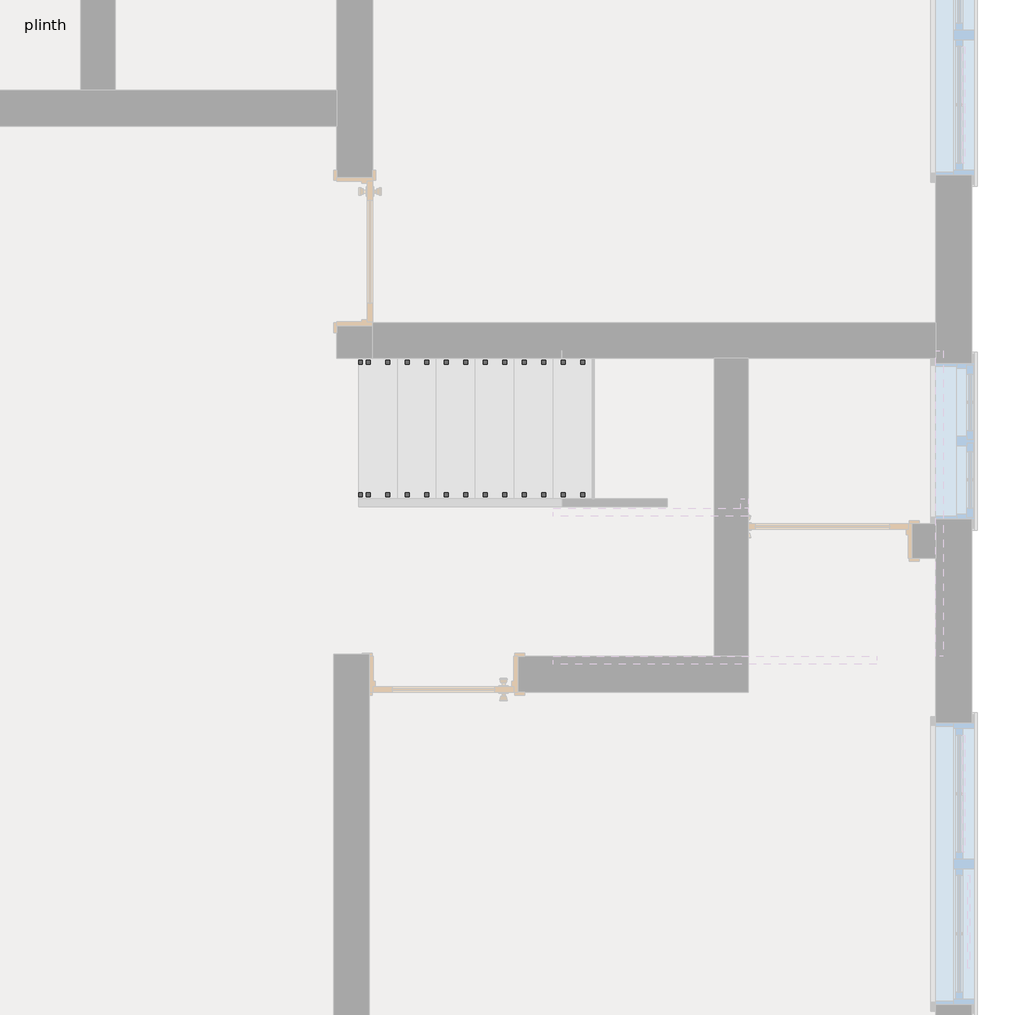
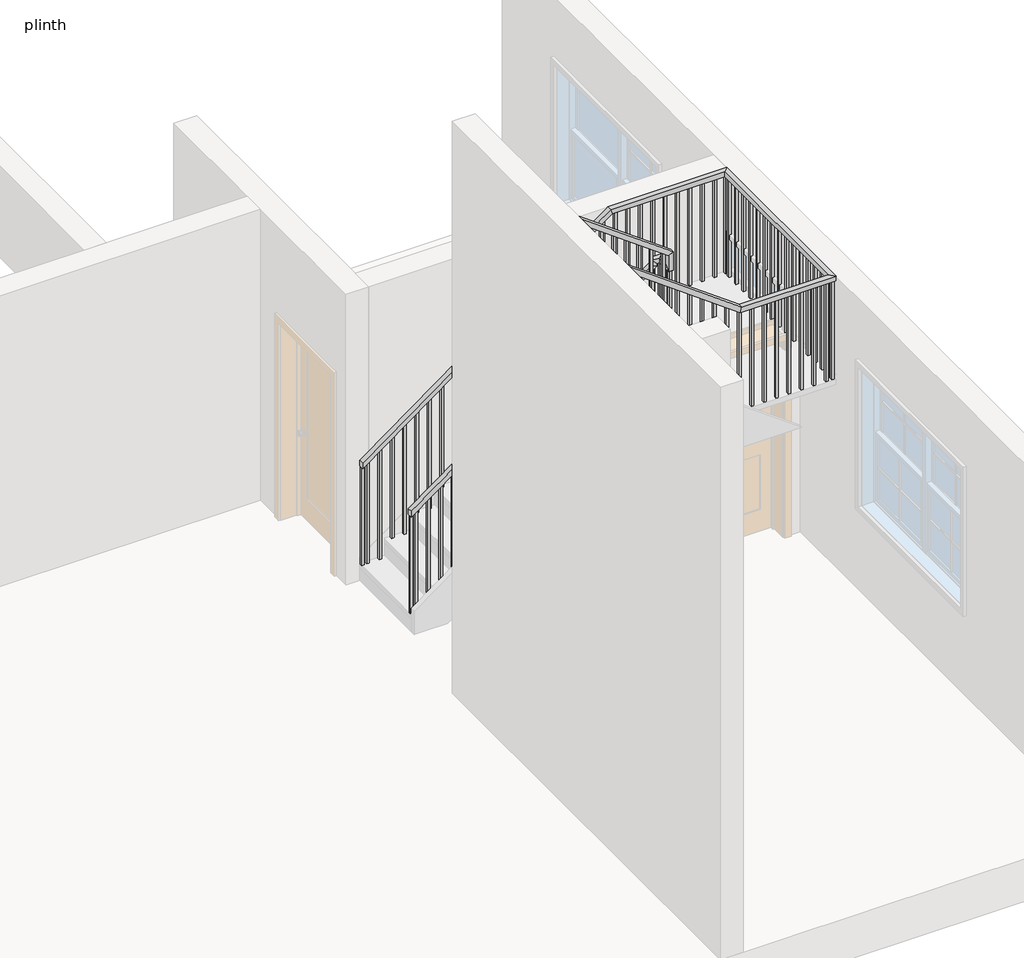
# One storey, part 2 of 3: 2 railings.
"""IFC4 building model written with IfcOpenShell, lengths in millimetres."""

from ifc_helpers import new_model, si_unit, frame, origin, place, context, project, spatial, polyline, outline, extrude, faceted_brep, element, save

model = new_model("IFC4")

# Units and contexts
model_context = context("Model", 3, world=origin())
ifc_project = project(units=[si_unit("LENGTHUNIT", "METRE", prefix="MILLI")], contexts=[model_context])

# Site, building, storey
site = spatial("IfcSite", under=ifc_project)
building = spatial("IfcBuilding", under=site)
storey = spatial("IfcBuildingStorey", under=building, Name="plinth", Elevation=450.0)

# Railings
placement = place(None, origin())
element("IfcRailing", 1, ObjectType="1100mm", at=placement, inside=storey, context=model_context, shape_type="SolidModel", body=[
    faceted_brep([(-8719.2253352, 6758.6914588, 1732.3529412), (-8719.2253352, 6758.6914588, 1670.4651087), (-8719.2253352, 6708.6914588, 1670.4651087), (-8719.2253352, 6708.6914588, 1732.3529412), (-6293.8253352, 6758.6914588, 3501.4682353), (-6243.8253352, 6758.6914588, 3476.0509911), (-6243.8253352, 6708.6914588, 3476.0509911), (-6293.8253352, 6708.6914588, 3501.4682353), (-6293.8253352, 6758.6914588, 3555.8823529), (-6243.8253352, 6758.6914588, 3505.8823529), (-6243.8253352, 6708.6914588, 3505.8823529), (-6293.8253352, 6708.6914588, 3555.8823529), (-6168.8253352, 6758.6914588, 3555.8823529), (-6168.8253352, 6758.6914588, 3505.8823529), (-6218.8253352, 6708.6914588, 3505.8823529), (-6218.8253352, 6708.6914588, 3555.8823529), (-6168.8253352, 6633.6914588, 3555.8823529), (-6168.8253352, 6633.6914588, 3505.8823529), (-6218.8253352, 6633.6914588, 3505.8823529), (-6218.8253352, 6633.6914588, 3555.8823529), (-6168.8253352, 6597.8914588, 3555.8823529), (-6218.8253352, 6597.8914588, 3555.8823529), (-6218.8253352, 6547.8914588, 3505.8823529), (-6168.8253352, 6547.8914588, 3505.8823529)], [[[0, 1, 2, 3]], [[1, 0, 4, 5]], [[2, 1, 5, 6]], [[3, 2, 6, 7]], [[0, 3, 7, 4]], [[5, 4, 8, 9]], [[6, 5, 9, 10]], [[7, 6, 10, 11]], [[4, 7, 11, 8]], [[9, 8, 12, 13]], [[10, 9, 13, 14]], [[11, 10, 14, 15]], [[8, 11, 15, 12]], [[13, 12, 16, 17]], [[14, 13, 17, 18]], [[15, 14, 18, 19]], [[12, 15, 19, 16]], [[20, 21, 22, 23]], [[17, 16, 20, 23]], [[18, 17, 23, 22]], [[19, 18, 22, 21]], [[16, 19, 21, 20]]]),
    faceted_brep([(-6168.8253352, 6597.8914588, 3555.8823529), (-6168.8253352, 6547.8914588, 3505.8823529), (-6218.8253352, 6547.8914588, 3505.8823529), (-6218.8253352, 6597.8914588, 3555.8823529), (-6168.8253352, 6597.8914588, 3701.4729412), (-6218.8253352, 6597.8914588, 3676.055697), (-6218.8253352, 6547.8914588, 3676.055697), (-6168.8253352, 6547.8914588, 3701.4729412)], [[[0, 1, 2, 3]], [[4, 5, 6, 7]], [[1, 0, 4, 7]], [[2, 1, 7, 6]], [[3, 2, 6, 5]], [[0, 3, 5, 4]]]),
    faceted_brep([(-6168.8253352, 6547.8914588, 3701.4729412), (-6218.8253352, 6547.8914588, 3676.055697), (-6218.8253352, 6597.8914588, 3676.055697), (-6168.8253352, 6597.8914588, 3701.4729412), (-7469.2253352, 6547.8914588, 4650.0), (-7469.2253352, 6597.8914588, 4650.0), (-7469.2253352, 6597.8914588, 4588.1121675), (-7469.2253352, 6547.8914588, 4588.1121675)], [[[0, 1, 2, 3]], [[4, 5, 6, 7]], [[1, 0, 4, 7]], [[2, 1, 7, 6]], [[3, 2, 6, 5]], [[0, 3, 5, 4]]]),
    extrude(outline(polyline([(3367.6470588, -7368.8253352), (4514.8792264, -7368.8253352), (4533.1145205, -7393.8253352), (3367.6470588, -7393.8253352), (3367.6470588, -7368.8253352)])), frame((0.0, 6560.3914588, 0.0), z_axis=(0.0, 1.0, 0.0), x_axis=(0.0, 0.0, 1.0)), (0.0, 0.0, 1.0), 25.0),
    extrude(outline(polyline([(3367.6470588, -7243.8253352), (4423.7027558, -7243.8253352), (4441.9380499, -7268.8253352), (3367.6470588, -7268.8253352), (3367.6470588, -7243.8253352)])), frame((0.0, 6560.3914588, 0.0), z_axis=(0.0, 1.0, 0.0), x_axis=(0.0, 0.0, 1.0)), (0.0, 0.0, 1.0), 25.0),
    extrude(outline(polyline([(3185.2941176, -7118.8253352), (4332.5262852, -7118.8253352), (4350.7615793, -7143.8253352), (3185.2941176, -7143.8253352), (3185.2941176, -7118.8253352)])), frame((0.0, 6560.3914588, 0.0), z_axis=(0.0, 1.0, 0.0), x_axis=(0.0, 0.0, 1.0)), (0.0, 0.0, 1.0), 25.0),
    extrude(outline(polyline([(3185.2941176, -6993.8253352), (4241.3498146, -6993.8253352), (4259.5851087, -7018.8253352), (3185.2941176, -7018.8253352), (3185.2941176, -6993.8253352)])), frame((0.0, 6560.3914588, 0.0), z_axis=(0.0, 1.0, 0.0), x_axis=(0.0, 0.0, 1.0)), (0.0, 0.0, 1.0), 25.0),
    extrude(outline(polyline([(3002.9411765, -6868.8253352), (4150.173344, -6868.8253352), (4168.4086381, -6893.8253352), (3002.9411765, -6893.8253352), (3002.9411765, -6868.8253352)])), frame((0.0, 6560.3914588, 0.0), z_axis=(0.0, 1.0, 0.0), x_axis=(0.0, 0.0, 1.0)), (0.0, 0.0, 1.0), 25.0),
    extrude(outline(polyline([(3002.9411765, -6743.8253352), (4058.9968734, -6743.8253352), (4077.2321675, -6768.8253352), (3002.9411765, -6768.8253352), (3002.9411765, -6743.8253352)])), frame((0.0, 6560.3914588, 0.0), z_axis=(0.0, 1.0, 0.0), x_axis=(0.0, 0.0, 1.0)), (0.0, 0.0, 1.0), 25.0),
    extrude(outline(polyline([(2820.5882353, -6618.8253352), (3967.8204028, -6618.8253352), (3986.055697, -6643.8253352), (2820.5882353, -6643.8253352), (2820.5882353, -6618.8253352)])), frame((0.0, 6560.3914588, 0.0), z_axis=(0.0, 1.0, 0.0), x_axis=(0.0, 0.0, 1.0)), (0.0, 0.0, 1.0), 25.0),
    extrude(outline(polyline([(2820.5882353, -6493.8253352), (3876.6439322, -6493.8253352), (3894.8792264, -6518.8253352), (2820.5882353, -6518.8253352), (2820.5882353, -6493.8253352)])), frame((0.0, 6560.3914588, 0.0), z_axis=(0.0, 1.0, 0.0), x_axis=(0.0, 0.0, 1.0)), (0.0, 0.0, 1.0), 25.0),
    extrude(outline(polyline([(2638.2352941, -6368.8253352), (3785.4674617, -6368.8253352), (3803.7027558, -6393.8253352), (2638.2352941, -6393.8253352), (2638.2352941, -6368.8253352)])), frame((0.0, 6560.3914588, 0.0), z_axis=(0.0, 1.0, 0.0), x_axis=(0.0, 0.0, 1.0)), (0.0, 0.0, 1.0), 25.0),
    extrude(outline(polyline([(2638.2352941, -6243.8253352), (3694.2909911, -6243.8253352), (3712.5262852, -6268.8253352), (2638.2352941, -6268.8253352), (2638.2352941, -6243.8253352)])), frame((0.0, 6560.3914588, 0.0), z_axis=(0.0, 1.0, 0.0), x_axis=(0.0, 0.0, 1.0)), (0.0, 0.0, 1.0), 25.0),
    extrude(outline(polyline([(-6206.3253352, 6683.6914588), (-6181.3253352, 6683.6914588), (-6181.3253352, 6658.6914588), (-6206.3253352, 6658.6914588), (-6206.3253352, 6683.6914588)])), frame((0.0, 0.0, 2455.8823529), z_axis=(0.0, 0.0, 1.0), x_axis=(1.0, 0.0, 0.0)), (0.0, 0.0, 1.0), 1050.0),
    extrude(outline(polyline([(-6294.2253352, 6721.1914588), (-6294.2253352, 6746.1914588), (-6269.2253352, 6746.1914588), (-6269.2253352, 6721.1914588), (-6294.2253352, 6721.1914588)])), frame((0.0, 0.0, 2273.5294118), z_axis=(0.0, 0.0, 1.0), x_axis=(1.0, 0.0, 0.0)), (0.0, 0.0, 1.0), 1232.3529412),
    extrude(outline(polyline([(3348.1121675, -6419.2253352), (2273.5294118, -6419.2253352), (2273.5294118, -6394.2253352), (3366.3474617, -6394.2253352), (3348.1121675, -6419.2253352)])), frame((0.0, 6721.1914588, 0.0), z_axis=(0.0, 1.0, 0.0), x_axis=(0.0, 0.0, 1.0)), (0.0, 0.0, 1.0), 25.0),
    extrude(outline(polyline([(3256.935697, -6544.2253352), (2091.1764706, -6544.2253352), (2091.1764706, -6519.2253352), (3275.1709911, -6519.2253352), (3256.935697, -6544.2253352)])), frame((0.0, 6721.1914588, 0.0), z_axis=(0.0, 1.0, 0.0), x_axis=(0.0, 0.0, 1.0)), (0.0, 0.0, 1.0), 25.0),
    extrude(outline(polyline([(3165.7592264, -6669.2253352), (2091.1764706, -6669.2253352), (2091.1764706, -6644.2253352), (3183.9945205, -6644.2253352), (3165.7592264, -6669.2253352)])), frame((0.0, 6721.1914588, 0.0), z_axis=(0.0, 1.0, 0.0), x_axis=(0.0, 0.0, 1.0)), (0.0, 0.0, 1.0), 25.0),
    extrude(outline(polyline([(3074.5827558, -6794.2253352), (1908.8235294, -6794.2253352), (1908.8235294, -6769.2253352), (3092.8180499, -6769.2253352), (3074.5827558, -6794.2253352)])), frame((0.0, 6721.1914588, 0.0), z_axis=(0.0, 1.0, 0.0), x_axis=(0.0, 0.0, 1.0)), (0.0, 0.0, 1.0), 25.0),
    extrude(outline(polyline([(2983.4062852, -6919.2253352), (1908.8235294, -6919.2253352), (1908.8235294, -6894.2253352), (3001.6415793, -6894.2253352), (2983.4062852, -6919.2253352)])), frame((0.0, 6721.1914588, 0.0), z_axis=(0.0, 1.0, 0.0), x_axis=(0.0, 0.0, 1.0)), (0.0, 0.0, 1.0), 25.0),
    extrude(outline(polyline([(2892.2298146, -7044.2253352), (1726.4705882, -7044.2253352), (1726.4705882, -7019.2253352), (2910.4651087, -7019.2253352), (2892.2298146, -7044.2253352)])), frame((0.0, 6721.1914588, 0.0), z_axis=(0.0, 1.0, 0.0), x_axis=(0.0, 0.0, 1.0)), (0.0, 0.0, 1.0), 25.0),
    extrude(outline(polyline([(2801.053344, -7169.2253352), (1726.4705882, -7169.2253352), (1726.4705882, -7144.2253352), (2819.2886381, -7144.2253352), (2801.053344, -7169.2253352)])), frame((0.0, 6721.1914588, 0.0), z_axis=(0.0, 1.0, 0.0), x_axis=(0.0, 0.0, 1.0)), (0.0, 0.0, 1.0), 25.0),
    extrude(outline(polyline([(2709.8768734, -7294.2253352), (1544.1176471, -7294.2253352), (1544.1176471, -7269.2253352), (2728.1121675, -7269.2253352), (2709.8768734, -7294.2253352)])), frame((0.0, 6721.1914588, 0.0), z_axis=(0.0, 1.0, 0.0), x_axis=(0.0, 0.0, 1.0)), (0.0, 0.0, 1.0), 25.0),
    extrude(outline(polyline([(2618.7004028, -7419.2253352), (1544.1176471, -7419.2253352), (1544.1176471, -7394.2253352), (2636.935697, -7394.2253352), (2618.7004028, -7419.2253352)])), frame((0.0, 6721.1914588, 0.0), z_axis=(0.0, 1.0, 0.0), x_axis=(0.0, 0.0, 1.0)), (0.0, 0.0, 1.0), 25.0),
    extrude(outline(polyline([(2527.5239322, -7544.2253352), (1361.7647059, -7544.2253352), (1361.7647059, -7519.2253352), (2545.7592264, -7519.2253352), (2527.5239322, -7544.2253352)])), frame((0.0, 6721.1914588, 0.0), z_axis=(0.0, 1.0, 0.0), x_axis=(0.0, 0.0, 1.0)), (0.0, 0.0, 1.0), 25.0),
    extrude(outline(polyline([(2436.3474617, -7669.2253352), (1361.7647059, -7669.2253352), (1361.7647059, -7644.2253352), (2454.5827558, -7644.2253352), (2436.3474617, -7669.2253352)])), frame((0.0, 6721.1914588, 0.0), z_axis=(0.0, 1.0, 0.0), x_axis=(0.0, 0.0, 1.0)), (0.0, 0.0, 1.0), 25.0),
    extrude(outline(polyline([(2345.1709911, -7794.2253352), (1179.4117647, -7794.2253352), (1179.4117647, -7769.2253352), (2363.4062852, -7769.2253352), (2345.1709911, -7794.2253352)])), frame((0.0, 6721.1914588, 0.0), z_axis=(0.0, 1.0, 0.0), x_axis=(0.0, 0.0, 1.0)), (0.0, 0.0, 1.0), 25.0),
    extrude(outline(polyline([(2253.9945205, -7919.2253352), (1179.4117647, -7919.2253352), (1179.4117647, -7894.2253352), (2272.2298146, -7894.2253352), (2253.9945205, -7919.2253352)])), frame((0.0, 6721.1914588, 0.0), z_axis=(0.0, 1.0, 0.0), x_axis=(0.0, 0.0, 1.0)), (0.0, 0.0, 1.0), 25.0),
    extrude(outline(polyline([(2162.8180499, -8044.2253352), (997.0588235, -8044.2253352), (997.0588235, -8019.2253352), (2181.053344, -8019.2253352), (2162.8180499, -8044.2253352)])), frame((0.0, 6721.1914588, 0.0), z_axis=(0.0, 1.0, 0.0), x_axis=(0.0, 0.0, 1.0)), (0.0, 0.0, 1.0), 25.0),
    extrude(outline(polyline([(2071.6415793, -8169.2253352), (997.0588235, -8169.2253352), (997.0588235, -8144.2253352), (2089.8768734, -8144.2253352), (2071.6415793, -8169.2253352)])), frame((0.0, 6721.1914588, 0.0), z_axis=(0.0, 1.0, 0.0), x_axis=(0.0, 0.0, 1.0)), (0.0, 0.0, 1.0), 25.0),
    extrude(outline(polyline([(1980.4651087, -8294.2253352), (814.7058824, -8294.2253352), (814.7058824, -8269.2253352), (1998.7004028, -8269.2253352), (1980.4651087, -8294.2253352)])), frame((0.0, 6721.1914588, 0.0), z_axis=(0.0, 1.0, 0.0), x_axis=(0.0, 0.0, 1.0)), (0.0, 0.0, 1.0), 25.0),
    extrude(outline(polyline([(1889.2886381, -8419.2253352), (814.7058824, -8419.2253352), (814.7058824, -8394.2253352), (1907.5239322, -8394.2253352), (1889.2886381, -8419.2253352)])), frame((0.0, 6721.1914588, 0.0), z_axis=(0.0, 1.0, 0.0), x_axis=(0.0, 0.0, 1.0)), (0.0, 0.0, 1.0), 25.0),
    extrude(outline(polyline([(1798.1121675, -8544.2253352), (632.3529412, -8544.2253352), (632.3529412, -8519.2253352), (1816.3474617, -8519.2253352), (1798.1121675, -8544.2253352)])), frame((0.0, 6721.1914588, 0.0), z_axis=(0.0, 1.0, 0.0), x_axis=(0.0, 0.0, 1.0)), (0.0, 0.0, 1.0), 25.0),
    extrude(outline(polyline([(1706.935697, -8669.2253352), (632.3529412, -8669.2253352), (632.3529412, -8644.2253352), (1725.1709911, -8644.2253352), (1706.935697, -8669.2253352)])), frame((0.0, 6721.1914588, 0.0), z_axis=(0.0, 1.0, 0.0), x_axis=(0.0, 0.0, 1.0)), (0.0, 0.0, 1.0), 25.0),
    extrude(outline(polyline([(-6206.3253352, 6585.3914588), (-6181.3253352, 6585.3914588), (-6181.3253352, 6560.3914588), (-6206.3253352, 6560.3914588), (-6206.3253352, 6585.3914588)])), frame((0.0, 0.0, 2455.8823529), z_axis=(0.0, 0.0, 1.0), x_axis=(1.0, 0.0, 0.0)), (0.0, 0.0, 1.0), 1050.0),
    extrude(outline(polyline([(-6206.3253352, 6721.1914588), (-6206.3253352, 6746.1914588), (-6181.3253352, 6746.1914588), (-6181.3253352, 6721.1914588), (-6206.3253352, 6721.1914588)])), frame((0.0, 0.0, 2455.8823529), z_axis=(0.0, 0.0, 1.0), x_axis=(1.0, 0.0, 0.0)), (0.0, 0.0, 1.0), 1050.0),
    extrude(outline(polyline([(3367.6470588, -7444.2253352), (4569.8768734, -7444.2253352), (4588.1121675, -7469.2253352), (3367.6470588, -7469.2253352), (3367.6470588, -7444.2253352)])), frame((0.0, 6560.3914588, 0.0), z_axis=(0.0, 1.0, 0.0), x_axis=(0.0, 0.0, 1.0)), (0.0, 0.0, 1.0), 25.0),
    extrude(outline(polyline([(1670.4651087, -8719.2253352), (632.3529412, -8719.2253352), (632.3529412, -8694.2253352), (1688.7004028, -8694.2253352), (1670.4651087, -8719.2253352)])), frame((0.0, 6721.1914588, 0.0), z_axis=(0.0, 1.0, 0.0), x_axis=(0.0, 0.0, 1.0)), (0.0, 0.0, 1.0), 25.0),
])
element("IfcRailing", 2, ObjectType="1100mm", at=placement, inside=storey, context=model_context, shape_type="SolidModel", body=[
    faceted_brep([(-8719.2253352, 7607.8914588, 1732.3529412), (-8719.2253352, 7607.8914588, 1670.4651087), (-8719.2253352, 7557.8914588, 1670.4651087), (-8719.2253352, 7557.8914588, 1732.3529412), (-6219.2253352, 7607.8914588, 3555.8823529), (-6202.9275004, 7607.8914588, 3505.8823529), (-6202.9275004, 7557.8914588, 3505.8823529), (-6219.2253352, 7557.8914588, 3555.8823529), (-5019.6253352, 7607.8914588, 3555.8823529), (-5019.6253352, 7607.8914588, 3505.8823529), (-5069.6253352, 7557.8914588, 3505.8823529), (-5069.6253352, 7557.8914588, 3555.8823529), (-5019.6253352, 5698.6914588, 3555.8823529), (-5019.6253352, 5698.6914588, 3505.8823529), (-5069.6253352, 5748.6914588, 3505.8823529), (-5069.6253352, 5748.6914588, 3555.8823529), (-5969.2253352, 5698.6914588, 3555.8823529), (-5985.52317, 5698.6914588, 3505.8823529), (-5985.52317, 5748.6914588, 3505.8823529), (-5969.2253352, 5748.6914588, 3555.8823529), (-7469.2253352, 5698.6914588, 4650.0), (-7469.2253352, 5748.6914588, 4650.0), (-7469.2253352, 5748.6914588, 4588.1121675), (-7469.2253352, 5698.6914588, 4588.1121675)], [[[0, 1, 2, 3]], [[1, 0, 4, 5]], [[2, 1, 5, 6]], [[3, 2, 6, 7]], [[0, 3, 7, 4]], [[5, 4, 8, 9]], [[6, 5, 9, 10]], [[7, 6, 10, 11]], [[4, 7, 11, 8]], [[9, 8, 12, 13]], [[10, 9, 13, 14]], [[11, 10, 14, 15]], [[8, 11, 15, 12]], [[13, 12, 16, 17]], [[14, 13, 17, 18]], [[15, 14, 18, 19]], [[12, 15, 19, 16]], [[20, 21, 22, 23]], [[17, 16, 20, 23]], [[18, 17, 23, 22]], [[19, 18, 22, 21]], [[16, 19, 21, 20]]]),
    extrude(outline(polyline([(4497.2274617, -7344.6253352), (4515.4627558, -7369.6253352), (3367.6470588, -7369.6253352), (3367.6470588, -7344.6253352), (4497.2274617, -7344.6253352)])), frame((0.0, 5711.1914588, 0.0), z_axis=(0.0, 1.0, 0.0), x_axis=(0.0, 0.0, 1.0)), (0.0, 0.0, 1.0), 25.0),
    extrude(outline(polyline([(4406.0509911, -7219.6253352), (4424.2862852, -7244.6253352), (3367.6470588, -7244.6253352), (3367.6470588, -7219.6253352), (4406.0509911, -7219.6253352)])), frame((0.0, 5711.1914588, 0.0), z_axis=(0.0, 1.0, 0.0), x_axis=(0.0, 0.0, 1.0)), (0.0, 0.0, 1.0), 25.0),
    extrude(outline(polyline([(4314.8745205, -7094.6253352), (4333.1098146, -7119.6253352), (3185.2941176, -7119.6253352), (3185.2941176, -7094.6253352), (4314.8745205, -7094.6253352)])), frame((0.0, 5711.1914588, 0.0), z_axis=(0.0, 1.0, 0.0), x_axis=(0.0, 0.0, 1.0)), (0.0, 0.0, 1.0), 25.0),
    extrude(outline(polyline([(4223.6980499, -6969.6253352), (4241.933344, -6994.6253352), (3185.2941176, -6994.6253352), (3185.2941176, -6969.6253352), (4223.6980499, -6969.6253352)])), frame((0.0, 5711.1914588, 0.0), z_axis=(0.0, 1.0, 0.0), x_axis=(0.0, 0.0, 1.0)), (0.0, 0.0, 1.0), 25.0),
    extrude(outline(polyline([(4132.5215793, -6844.6253352), (4150.7568734, -6869.6253352), (3002.9411765, -6869.6253352), (3002.9411765, -6844.6253352), (4132.5215793, -6844.6253352)])), frame((0.0, 5711.1914588, 0.0), z_axis=(0.0, 1.0, 0.0), x_axis=(0.0, 0.0, 1.0)), (0.0, 0.0, 1.0), 25.0),
    extrude(outline(polyline([(4041.3451087, -6719.6253352), (4059.5804028, -6744.6253352), (3002.9411765, -6744.6253352), (3002.9411765, -6719.6253352), (4041.3451087, -6719.6253352)])), frame((0.0, 5711.1914588, 0.0), z_axis=(0.0, 1.0, 0.0), x_axis=(0.0, 0.0, 1.0)), (0.0, 0.0, 1.0), 25.0),
    extrude(outline(polyline([(3950.1686381, -6594.6253352), (3968.4039322, -6619.6253352), (2820.5882353, -6619.6253352), (2820.5882353, -6594.6253352), (3950.1686381, -6594.6253352)])), frame((0.0, 5711.1914588, 0.0), z_axis=(0.0, 1.0, 0.0), x_axis=(0.0, 0.0, 1.0)), (0.0, 0.0, 1.0), 25.0),
    extrude(outline(polyline([(3858.9921675, -6469.6253352), (3877.2274617, -6494.6253352), (2820.5882353, -6494.6253352), (2820.5882353, -6469.6253352), (3858.9921675, -6469.6253352)])), frame((0.0, 5711.1914588, 0.0), z_axis=(0.0, 1.0, 0.0), x_axis=(0.0, 0.0, 1.0)), (0.0, 0.0, 1.0), 25.0),
    extrude(outline(polyline([(3767.815697, -6344.6253352), (3786.0509911, -6369.6253352), (2638.2352941, -6369.6253352), (2638.2352941, -6344.6253352), (3767.815697, -6344.6253352)])), frame((0.0, 5711.1914588, 0.0), z_axis=(0.0, 1.0, 0.0), x_axis=(0.0, 0.0, 1.0)), (0.0, 0.0, 1.0), 25.0),
    extrude(outline(polyline([(3676.6392264, -6219.6253352), (3694.8745205, -6244.6253352), (2638.2352941, -6244.6253352), (2638.2352941, -6219.6253352), (3676.6392264, -6219.6253352)])), frame((0.0, 5711.1914588, 0.0), z_axis=(0.0, 1.0, 0.0), x_axis=(0.0, 0.0, 1.0)), (0.0, 0.0, 1.0), 25.0),
    extrude(outline(polyline([(3585.4627558, -6094.6253352), (3603.6980499, -6119.6253352), (2455.8823529, -6119.6253352), (2455.8823529, -6094.6253352), (3585.4627558, -6094.6253352)])), frame((0.0, 5711.1914588, 0.0), z_axis=(0.0, 1.0, 0.0), x_axis=(0.0, 0.0, 1.0)), (0.0, 0.0, 1.0), 25.0),
    extrude(outline(polyline([(3494.2862852, -5969.6253352), (3512.5215793, -5994.6253352), (2455.8823529, -5994.6253352), (2455.8823529, -5969.6253352), (3494.2862852, -5969.6253352)])), frame((0.0, 5711.1914588, 0.0), z_axis=(0.0, 1.0, 0.0), x_axis=(0.0, 0.0, 1.0)), (0.0, 0.0, 1.0), 25.0),
    extrude(outline(polyline([(-5844.6253352, 5711.1914588), (-5869.6253352, 5711.1914588), (-5869.6253352, 5736.1914588), (-5844.6253352, 5736.1914588), (-5844.6253352, 5711.1914588)])), frame((0.0, 0.0, 2455.8823529), z_axis=(0.0, 0.0, 1.0), x_axis=(1.0, 0.0, 0.0)), (0.0, 0.0, 1.0), 1050.0),
    extrude(outline(polyline([(-5719.6253352, 5711.1914588), (-5744.6253352, 5711.1914588), (-5744.6253352, 5736.1914588), (-5719.6253352, 5736.1914588), (-5719.6253352, 5711.1914588)])), frame((0.0, 0.0, 2455.8823529), z_axis=(0.0, 0.0, 1.0), x_axis=(1.0, 0.0, 0.0)), (0.0, 0.0, 1.0), 1050.0),
    extrude(outline(polyline([(-5594.6253352, 5711.1914588), (-5619.6253352, 5711.1914588), (-5619.6253352, 5736.1914588), (-5594.6253352, 5736.1914588), (-5594.6253352, 5711.1914588)])), frame((0.0, 0.0, 2455.8823529), z_axis=(0.0, 0.0, 1.0), x_axis=(1.0, 0.0, 0.0)), (0.0, 0.0, 1.0), 1050.0),
    extrude(outline(polyline([(-5469.6253352, 5711.1914588), (-5494.6253352, 5711.1914588), (-5494.6253352, 5736.1914588), (-5469.6253352, 5736.1914588), (-5469.6253352, 5711.1914588)])), frame((0.0, 0.0, 2455.8823529), z_axis=(0.0, 0.0, 1.0), x_axis=(1.0, 0.0, 0.0)), (0.0, 0.0, 1.0), 1050.0),
    extrude(outline(polyline([(-5344.6253352, 5711.1914588), (-5369.6253352, 5711.1914588), (-5369.6253352, 5736.1914588), (-5344.6253352, 5736.1914588), (-5344.6253352, 5711.1914588)])), frame((0.0, 0.0, 2455.8823529), z_axis=(0.0, 0.0, 1.0), x_axis=(1.0, 0.0, 0.0)), (0.0, 0.0, 1.0), 1050.0),
    extrude(outline(polyline([(-5219.6253352, 5711.1914588), (-5244.6253352, 5711.1914588), (-5244.6253352, 5736.1914588), (-5219.6253352, 5736.1914588), (-5219.6253352, 5711.1914588)])), frame((0.0, 0.0, 2455.8823529), z_axis=(0.0, 0.0, 1.0), x_axis=(1.0, 0.0, 0.0)), (0.0, 0.0, 1.0), 1050.0),
    extrude(outline(polyline([(-5094.6253352, 5711.1914588), (-5119.6253352, 5711.1914588), (-5119.6253352, 5736.1914588), (-5094.6253352, 5736.1914588), (-5094.6253352, 5711.1914588)])), frame((0.0, 0.0, 2455.8823529), z_axis=(0.0, 0.0, 1.0), x_axis=(1.0, 0.0, 0.0)), (0.0, 0.0, 1.0), 1050.0),
    extrude(outline(polyline([(-5032.1253352, 5782.8914588), (-5032.1253352, 5757.8914588), (-5057.1253352, 5757.8914588), (-5057.1253352, 5782.8914588), (-5032.1253352, 5782.8914588)])), frame((0.0, 0.0, 2455.8823529), z_axis=(0.0, 0.0, 1.0), x_axis=(1.0, 0.0, 0.0)), (0.0, 0.0, 1.0), 1050.0),
    extrude(outline(polyline([(-5032.1253352, 5907.8914588), (-5032.1253352, 5882.8914588), (-5057.1253352, 5882.8914588), (-5057.1253352, 5907.8914588), (-5032.1253352, 5907.8914588)])), frame((0.0, 0.0, 2455.8823529), z_axis=(0.0, 0.0, 1.0), x_axis=(1.0, 0.0, 0.0)), (0.0, 0.0, 1.0), 1050.0),
    extrude(outline(polyline([(-5032.1253352, 6032.8914588), (-5032.1253352, 6007.8914588), (-5057.1253352, 6007.8914588), (-5057.1253352, 6032.8914588), (-5032.1253352, 6032.8914588)])), frame((0.0, 0.0, 2455.8823529), z_axis=(0.0, 0.0, 1.0), x_axis=(1.0, 0.0, 0.0)), (0.0, 0.0, 1.0), 1050.0),
    extrude(outline(polyline([(-5032.1253352, 6157.8914588), (-5032.1253352, 6132.8914588), (-5057.1253352, 6132.8914588), (-5057.1253352, 6157.8914588), (-5032.1253352, 6157.8914588)])), frame((0.0, 0.0, 2455.8823529), z_axis=(0.0, 0.0, 1.0), x_axis=(1.0, 0.0, 0.0)), (0.0, 0.0, 1.0), 1050.0),
    extrude(outline(polyline([(-5032.1253352, 6282.8914588), (-5032.1253352, 6257.8914588), (-5057.1253352, 6257.8914588), (-5057.1253352, 6282.8914588), (-5032.1253352, 6282.8914588)])), frame((0.0, 0.0, 2455.8823529), z_axis=(0.0, 0.0, 1.0), x_axis=(1.0, 0.0, 0.0)), (0.0, 0.0, 1.0), 1050.0),
    extrude(outline(polyline([(-5032.1253352, 6407.8914588), (-5032.1253352, 6382.8914588), (-5057.1253352, 6382.8914588), (-5057.1253352, 6407.8914588), (-5032.1253352, 6407.8914588)])), frame((0.0, 0.0, 2455.8823529), z_axis=(0.0, 0.0, 1.0), x_axis=(1.0, 0.0, 0.0)), (0.0, 0.0, 1.0), 1050.0),
    extrude(outline(polyline([(-5032.1253352, 6532.8914588), (-5032.1253352, 6507.8914588), (-5057.1253352, 6507.8914588), (-5057.1253352, 6532.8914588), (-5032.1253352, 6532.8914588)])), frame((0.0, 0.0, 2455.8823529), z_axis=(0.0, 0.0, 1.0), x_axis=(1.0, 0.0, 0.0)), (0.0, 0.0, 1.0), 1050.0),
    extrude(outline(polyline([(-5032.1253352, 6657.8914588), (-5032.1253352, 6632.8914588), (-5057.1253352, 6632.8914588), (-5057.1253352, 6657.8914588), (-5032.1253352, 6657.8914588)])), frame((0.0, 0.0, 2455.8823529), z_axis=(0.0, 0.0, 1.0), x_axis=(1.0, 0.0, 0.0)), (0.0, 0.0, 1.0), 1050.0),
    extrude(outline(polyline([(-5032.1253352, 6782.8914588), (-5032.1253352, 6757.8914588), (-5057.1253352, 6757.8914588), (-5057.1253352, 6782.8914588), (-5032.1253352, 6782.8914588)])), frame((0.0, 0.0, 2455.8823529), z_axis=(0.0, 0.0, 1.0), x_axis=(1.0, 0.0, 0.0)), (0.0, 0.0, 1.0), 1050.0),
    extrude(outline(polyline([(-5032.1253352, 6907.8914588), (-5032.1253352, 6882.8914588), (-5057.1253352, 6882.8914588), (-5057.1253352, 6907.8914588), (-5032.1253352, 6907.8914588)])), frame((0.0, 0.0, 2455.8823529), z_axis=(0.0, 0.0, 1.0), x_axis=(1.0, 0.0, 0.0)), (0.0, 0.0, 1.0), 1050.0),
    extrude(outline(polyline([(-5032.1253352, 7032.8914588), (-5032.1253352, 7007.8914588), (-5057.1253352, 7007.8914588), (-5057.1253352, 7032.8914588), (-5032.1253352, 7032.8914588)])), frame((0.0, 0.0, 2455.8823529), z_axis=(0.0, 0.0, 1.0), x_axis=(1.0, 0.0, 0.0)), (0.0, 0.0, 1.0), 1050.0),
    extrude(outline(polyline([(-5032.1253352, 7157.8914588), (-5032.1253352, 7132.8914588), (-5057.1253352, 7132.8914588), (-5057.1253352, 7157.8914588), (-5032.1253352, 7157.8914588)])), frame((0.0, 0.0, 2455.8823529), z_axis=(0.0, 0.0, 1.0), x_axis=(1.0, 0.0, 0.0)), (0.0, 0.0, 1.0), 1050.0),
    extrude(outline(polyline([(-5032.1253352, 7282.8914588), (-5032.1253352, 7257.8914588), (-5057.1253352, 7257.8914588), (-5057.1253352, 7282.8914588), (-5032.1253352, 7282.8914588)])), frame((0.0, 0.0, 2455.8823529), z_axis=(0.0, 0.0, 1.0), x_axis=(1.0, 0.0, 0.0)), (0.0, 0.0, 1.0), 1050.0),
    extrude(outline(polyline([(-5032.1253352, 7407.8914588), (-5032.1253352, 7382.8914588), (-5057.1253352, 7382.8914588), (-5057.1253352, 7407.8914588), (-5032.1253352, 7407.8914588)])), frame((0.0, 0.0, 2455.8823529), z_axis=(0.0, 0.0, 1.0), x_axis=(1.0, 0.0, 0.0)), (0.0, 0.0, 1.0), 1050.0),
    extrude(outline(polyline([(-5032.1253352, 7532.8914588), (-5032.1253352, 7507.8914588), (-5057.1253352, 7507.8914588), (-5057.1253352, 7532.8914588), (-5032.1253352, 7532.8914588)])), frame((0.0, 0.0, 2455.8823529), z_axis=(0.0, 0.0, 1.0), x_axis=(1.0, 0.0, 0.0)), (0.0, 0.0, 1.0), 1050.0),
    extrude(outline(polyline([(-5169.2253352, 7595.3914588), (-5144.2253352, 7595.3914588), (-5144.2253352, 7570.3914588), (-5169.2253352, 7570.3914588), (-5169.2253352, 7595.3914588)])), frame((0.0, 0.0, 2455.8823529), z_axis=(0.0, 0.0, 1.0), x_axis=(1.0, 0.0, 0.0)), (0.0, 0.0, 1.0), 1050.0),
    extrude(outline(polyline([(-5294.2253352, 7595.3914588), (-5269.2253352, 7595.3914588), (-5269.2253352, 7570.3914588), (-5294.2253352, 7570.3914588), (-5294.2253352, 7595.3914588)])), frame((0.0, 0.0, 2455.8823529), z_axis=(0.0, 0.0, 1.0), x_axis=(1.0, 0.0, 0.0)), (0.0, 0.0, 1.0), 1050.0),
    extrude(outline(polyline([(-5419.2253352, 7595.3914588), (-5394.2253352, 7595.3914588), (-5394.2253352, 7570.3914588), (-5419.2253352, 7570.3914588), (-5419.2253352, 7595.3914588)])), frame((0.0, 0.0, 2455.8823529), z_axis=(0.0, 0.0, 1.0), x_axis=(1.0, 0.0, 0.0)), (0.0, 0.0, 1.0), 1050.0),
    extrude(outline(polyline([(-5544.2253352, 7595.3914588), (-5519.2253352, 7595.3914588), (-5519.2253352, 7570.3914588), (-5544.2253352, 7570.3914588), (-5544.2253352, 7595.3914588)])), frame((0.0, 0.0, 2455.8823529), z_axis=(0.0, 0.0, 1.0), x_axis=(1.0, 0.0, 0.0)), (0.0, 0.0, 1.0), 1050.0),
    extrude(outline(polyline([(-5669.2253352, 7595.3914588), (-5644.2253352, 7595.3914588), (-5644.2253352, 7570.3914588), (-5669.2253352, 7570.3914588), (-5669.2253352, 7595.3914588)])), frame((0.0, 0.0, 2455.8823529), z_axis=(0.0, 0.0, 1.0), x_axis=(1.0, 0.0, 0.0)), (0.0, 0.0, 1.0), 1050.0),
    extrude(outline(polyline([(-5794.2253352, 7595.3914588), (-5769.2253352, 7595.3914588), (-5769.2253352, 7570.3914588), (-5794.2253352, 7570.3914588), (-5794.2253352, 7595.3914588)])), frame((0.0, 0.0, 2455.8823529), z_axis=(0.0, 0.0, 1.0), x_axis=(1.0, 0.0, 0.0)), (0.0, 0.0, 1.0), 1050.0),
    extrude(outline(polyline([(-5919.2253352, 7595.3914588), (-5894.2253352, 7595.3914588), (-5894.2253352, 7570.3914588), (-5919.2253352, 7570.3914588), (-5919.2253352, 7595.3914588)])), frame((0.0, 0.0, 2455.8823529), z_axis=(0.0, 0.0, 1.0), x_axis=(1.0, 0.0, 0.0)), (0.0, 0.0, 1.0), 1050.0),
    extrude(outline(polyline([(-6044.2253352, 7595.3914588), (-6019.2253352, 7595.3914588), (-6019.2253352, 7570.3914588), (-6044.2253352, 7570.3914588), (-6044.2253352, 7595.3914588)])), frame((0.0, 0.0, 2455.8823529), z_axis=(0.0, 0.0, 1.0), x_axis=(1.0, 0.0, 0.0)), (0.0, 0.0, 1.0), 1050.0),
    extrude(outline(polyline([(-6169.2253352, 7595.3914588), (-6144.2253352, 7595.3914588), (-6144.2253352, 7570.3914588), (-6169.2253352, 7570.3914588), (-6169.2253352, 7595.3914588)])), frame((0.0, 0.0, 2455.8823529), z_axis=(0.0, 0.0, 1.0), x_axis=(1.0, 0.0, 0.0)), (0.0, 0.0, 1.0), 1050.0),
    extrude(outline(polyline([(2273.5294118, -6294.2253352), (2273.5294118, -6269.2253352), (3457.5239322, -6269.2253352), (3439.2886381, -6294.2253352), (2273.5294118, -6294.2253352)])), frame((0.0, 7570.3914588, 0.0), z_axis=(0.0, 1.0, 0.0), x_axis=(0.0, 0.0, 1.0)), (0.0, 0.0, 1.0), 25.0),
    extrude(outline(polyline([(2273.5294118, -6419.2253352), (2273.5294118, -6394.2253352), (3366.3474617, -6394.2253352), (3348.1121675, -6419.2253352), (2273.5294118, -6419.2253352)])), frame((0.0, 7570.3914588, 0.0), z_axis=(0.0, 1.0, 0.0), x_axis=(0.0, 0.0, 1.0)), (0.0, 0.0, 1.0), 25.0),
    extrude(outline(polyline([(2091.1764706, -6544.2253352), (2091.1764706, -6519.2253352), (3275.1709911, -6519.2253352), (3256.935697, -6544.2253352), (2091.1764706, -6544.2253352)])), frame((0.0, 7570.3914588, 0.0), z_axis=(0.0, 1.0, 0.0), x_axis=(0.0, 0.0, 1.0)), (0.0, 0.0, 1.0), 25.0),
    extrude(outline(polyline([(2091.1764706, -6669.2253352), (2091.1764706, -6644.2253352), (3183.9945205, -6644.2253352), (3165.7592264, -6669.2253352), (2091.1764706, -6669.2253352)])), frame((0.0, 7570.3914588, 0.0), z_axis=(0.0, 1.0, 0.0), x_axis=(0.0, 0.0, 1.0)), (0.0, 0.0, 1.0), 25.0),
    extrude(outline(polyline([(1908.8235294, -6794.2253352), (1908.8235294, -6769.2253352), (3092.8180499, -6769.2253352), (3074.5827558, -6794.2253352), (1908.8235294, -6794.2253352)])), frame((0.0, 7570.3914588, 0.0), z_axis=(0.0, 1.0, 0.0), x_axis=(0.0, 0.0, 1.0)), (0.0, 0.0, 1.0), 25.0),
    extrude(outline(polyline([(1908.8235294, -6919.2253352), (1908.8235294, -6894.2253352), (3001.6415793, -6894.2253352), (2983.4062852, -6919.2253352), (1908.8235294, -6919.2253352)])), frame((0.0, 7570.3914588, 0.0), z_axis=(0.0, 1.0, 0.0), x_axis=(0.0, 0.0, 1.0)), (0.0, 0.0, 1.0), 25.0),
    extrude(outline(polyline([(1726.4705882, -7044.2253352), (1726.4705882, -7019.2253352), (2910.4651087, -7019.2253352), (2892.2298146, -7044.2253352), (1726.4705882, -7044.2253352)])), frame((0.0, 7570.3914588, 0.0), z_axis=(0.0, 1.0, 0.0), x_axis=(0.0, 0.0, 1.0)), (0.0, 0.0, 1.0), 25.0),
    extrude(outline(polyline([(1726.4705882, -7169.2253352), (1726.4705882, -7144.2253352), (2819.2886381, -7144.2253352), (2801.053344, -7169.2253352), (1726.4705882, -7169.2253352)])), frame((0.0, 7570.3914588, 0.0), z_axis=(0.0, 1.0, 0.0), x_axis=(0.0, 0.0, 1.0)), (0.0, 0.0, 1.0), 25.0),
    extrude(outline(polyline([(1544.1176471, -7294.2253352), (1544.1176471, -7269.2253352), (2728.1121675, -7269.2253352), (2709.8768734, -7294.2253352), (1544.1176471, -7294.2253352)])), frame((0.0, 7570.3914588, 0.0), z_axis=(0.0, 1.0, 0.0), x_axis=(0.0, 0.0, 1.0)), (0.0, 0.0, 1.0), 25.0),
    extrude(outline(polyline([(1544.1176471, -7419.2253352), (1544.1176471, -7394.2253352), (2636.935697, -7394.2253352), (2618.7004028, -7419.2253352), (1544.1176471, -7419.2253352)])), frame((0.0, 7570.3914588, 0.0), z_axis=(0.0, 1.0, 0.0), x_axis=(0.0, 0.0, 1.0)), (0.0, 0.0, 1.0), 25.0),
    extrude(outline(polyline([(1361.7647059, -7544.2253352), (1361.7647059, -7519.2253352), (2545.7592264, -7519.2253352), (2527.5239322, -7544.2253352), (1361.7647059, -7544.2253352)])), frame((0.0, 7570.3914588, 0.0), z_axis=(0.0, 1.0, 0.0), x_axis=(0.0, 0.0, 1.0)), (0.0, 0.0, 1.0), 25.0),
    extrude(outline(polyline([(1361.7647059, -7669.2253352), (1361.7647059, -7644.2253352), (2454.5827558, -7644.2253352), (2436.3474617, -7669.2253352), (1361.7647059, -7669.2253352)])), frame((0.0, 7570.3914588, 0.0), z_axis=(0.0, 1.0, 0.0), x_axis=(0.0, 0.0, 1.0)), (0.0, 0.0, 1.0), 25.0),
    extrude(outline(polyline([(1179.4117647, -7794.2253352), (1179.4117647, -7769.2253352), (2363.4062852, -7769.2253352), (2345.1709911, -7794.2253352), (1179.4117647, -7794.2253352)])), frame((0.0, 7570.3914588, 0.0), z_axis=(0.0, 1.0, 0.0), x_axis=(0.0, 0.0, 1.0)), (0.0, 0.0, 1.0), 25.0),
    extrude(outline(polyline([(1179.4117647, -7919.2253352), (1179.4117647, -7894.2253352), (2272.2298146, -7894.2253352), (2253.9945205, -7919.2253352), (1179.4117647, -7919.2253352)])), frame((0.0, 7570.3914588, 0.0), z_axis=(0.0, 1.0, 0.0), x_axis=(0.0, 0.0, 1.0)), (0.0, 0.0, 1.0), 25.0),
    extrude(outline(polyline([(997.0588235, -8044.2253352), (997.0588235, -8019.2253352), (2181.053344, -8019.2253352), (2162.8180499, -8044.2253352), (997.0588235, -8044.2253352)])), frame((0.0, 7570.3914588, 0.0), z_axis=(0.0, 1.0, 0.0), x_axis=(0.0, 0.0, 1.0)), (0.0, 0.0, 1.0), 25.0),
    extrude(outline(polyline([(997.0588235, -8169.2253352), (997.0588235, -8144.2253352), (2089.8768734, -8144.2253352), (2071.6415793, -8169.2253352), (997.0588235, -8169.2253352)])), frame((0.0, 7570.3914588, 0.0), z_axis=(0.0, 1.0, 0.0), x_axis=(0.0, 0.0, 1.0)), (0.0, 0.0, 1.0), 25.0),
    extrude(outline(polyline([(814.7058824, -8294.2253352), (814.7058824, -8269.2253352), (1998.7004028, -8269.2253352), (1980.4651087, -8294.2253352), (814.7058824, -8294.2253352)])), frame((0.0, 7570.3914588, 0.0), z_axis=(0.0, 1.0, 0.0), x_axis=(0.0, 0.0, 1.0)), (0.0, 0.0, 1.0), 25.0),
    extrude(outline(polyline([(814.7058824, -8419.2253352), (814.7058824, -8394.2253352), (1907.5239322, -8394.2253352), (1889.2886381, -8419.2253352), (814.7058824, -8419.2253352)])), frame((0.0, 7570.3914588, 0.0), z_axis=(0.0, 1.0, 0.0), x_axis=(0.0, 0.0, 1.0)), (0.0, 0.0, 1.0), 25.0),
    extrude(outline(polyline([(632.3529412, -8544.2253352), (632.3529412, -8519.2253352), (1816.3474617, -8519.2253352), (1798.1121675, -8544.2253352), (632.3529412, -8544.2253352)])), frame((0.0, 7570.3914588, 0.0), z_axis=(0.0, 1.0, 0.0), x_axis=(0.0, 0.0, 1.0)), (0.0, 0.0, 1.0), 25.0),
    extrude(outline(polyline([(632.3529412, -8669.2253352), (632.3529412, -8644.2253352), (1725.1709911, -8644.2253352), (1706.935697, -8669.2253352), (632.3529412, -8669.2253352)])), frame((0.0, 7570.3914588, 0.0), z_axis=(0.0, 1.0, 0.0), x_axis=(0.0, 0.0, 1.0)), (0.0, 0.0, 1.0), 25.0),
    extrude(outline(polyline([(-5032.1253352, 5736.1914588), (-5032.1253352, 5711.1914588), (-5057.1253352, 5711.1914588), (-5057.1253352, 5736.1914588), (-5032.1253352, 5736.1914588)])), frame((0.0, 0.0, 2455.8823529), z_axis=(0.0, 0.0, 1.0), x_axis=(1.0, 0.0, 0.0)), (0.0, 0.0, 1.0), 1050.0),
    extrude(outline(polyline([(-5057.1253352, 7595.3914588), (-5032.1253352, 7595.3914588), (-5032.1253352, 7570.3914588), (-5057.1253352, 7570.3914588), (-5057.1253352, 7595.3914588)])), frame((0.0, 0.0, 2455.8823529), z_axis=(0.0, 0.0, 1.0), x_axis=(1.0, 0.0, 0.0)), (0.0, 0.0, 1.0), 1050.0),
    extrude(outline(polyline([(4569.8768734, -7444.2253352), (4588.1121675, -7469.2253352), (3367.6470588, -7469.2253352), (3367.6470588, -7444.2253352), (4569.8768734, -7444.2253352)])), frame((0.0, 5711.1914588, 0.0), z_axis=(0.0, 1.0, 0.0), x_axis=(0.0, 0.0, 1.0)), (0.0, 0.0, 1.0), 25.0),
    extrude(outline(polyline([(632.3529412, -8719.2253352), (632.3529412, -8694.2253352), (1688.7004028, -8694.2253352), (1670.4651087, -8719.2253352), (632.3529412, -8719.2253352)])), frame((0.0, 7570.3914588, 0.0), z_axis=(0.0, 1.0, 0.0), x_axis=(0.0, 0.0, 1.0)), (0.0, 0.0, 1.0), 25.0),
])

save(model, "model.ifc")

# Revit data of these elements
# Project information
#   Project Issue Date = "Issue Date"
#   Project Status = "Project Status"
#   Client Name = "Owner"
#   Project Address = "Enter address here"
#   Project Name = "Project Name"
#   Project Number = "0001"
# Type "1100mm"
#   built-in parameter 1008612 = 0.019685 (stored number, unit not read)
#   built-in parameter 1008611 = 0.019685 (stored number, unit not read)
#   built-in parameter 1008609 = 0.902231 (stored number, unit not read)
#   built-in parameter 1008604 = 0.19685 (stored number, unit not read)
#   built-in parameter 1008603 = 0.164042 (stored number, unit not read)
#   Railing Height = 110 cm
#   built-in parameter 1008630 = 2
#   built-in parameter 1008610 = 2
#   built-in parameter 1008608 = 1
#   built-in parameter 1008618 = M_Baluster - Square : 25mm
# Elements 1, 2 (IfcRailing, "1100mm")
#   Phase Created = New Construction
